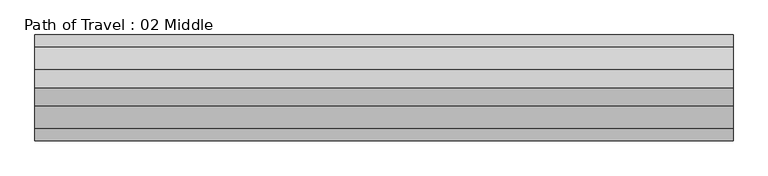
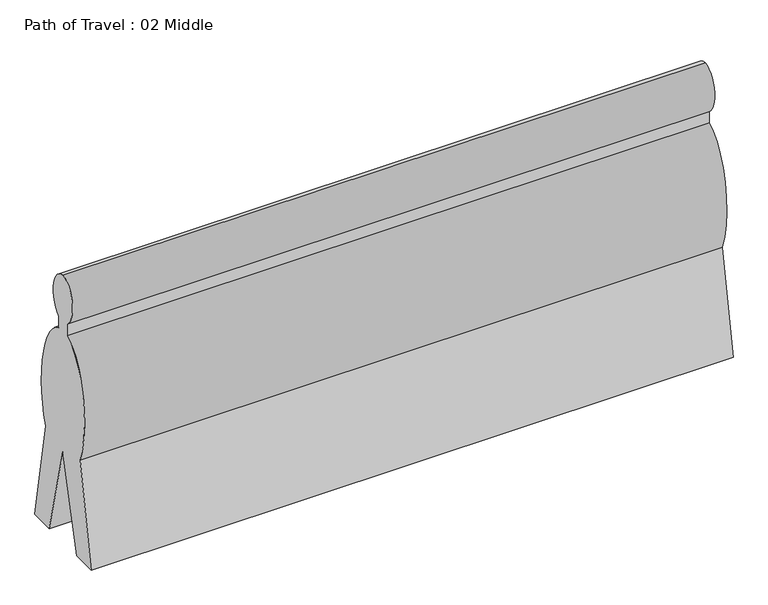
"""IFC4 building model written with IfcOpenShell, lengths in millimetres: proxy geometry, Path of Travel : 02 Middle."""

import ifcopenshell
import ifcopenshell.guid

model = None  # the IFC model being written
_history = None  # IfcOwnerHistory: only IFC2X3 demands one
_inside = {}  # id of a spatial element -> (the spatial element, [elements in it])
_under = {}  # id of a project, library or spatial element -> (it, [spatial elements below it])
_declared = {}  # id of a project -> (the project, [libraries it declares])
_typed = {}  # id of a type object -> (the type object, [elements of that type])
_made_of = {}  # id of a material, layer set ... -> (it, [elements and type objects made of it])


def new_model(schema):
    """Start an empty IFC model of exactly this schema.

    Asked for "IFC4X3", IfcOpenShell would pick the latest addendum, in which some entities
    have other attributes; the version numbers below select the first issue.
    IFC2X3 requires an IfcOwnerHistory on every rooted entity: one is made here for all.
    """
    global model, _history
    if schema == "IFC4X3":
        model = ifcopenshell.file(schema_version=(4, 3, 0, 0))
    else:
        model = ifcopenshell.file(schema=schema)
    _inside.clear()
    _under.clear()
    _declared.clear()
    _typed.clear()
    _made_of.clear()
    _history = None
    if model.schema == "IFC2X3":
        org = make("IfcOrganization", Name="unknown")
        user = make(
            "IfcPersonAndOrganization",
            ThePerson=make("IfcPerson", FamilyName="unknown"),
            TheOrganization=org,
        )
        app = make(
            "IfcApplication",
            ApplicationDeveloper=org,
            Version="unknown",
            ApplicationFullName="unknown",
            ApplicationIdentifier="unknown",
        )
        _history = make(
            "IfcOwnerHistory",
            OwningUser=user,
            OwningApplication=app,
            ChangeAction="ADDED",
            CreationDate=0,
        )
    return model


def make(cls, **values):
    """One entity of the class cls with the attributes given. An attribute that is None is left unset."""
    return model.create_entity(
        cls, **{name: value for name, value in values.items() if value is not None}
    )


def rooted(cls, **values):
    """An entity with a GlobalId (a new one), such as an element, a storey or a relation."""
    return make(cls, GlobalId=ifcopenshell.guid.new(), OwnerHistory=_history, **values)


def si_unit(unit_type, name, prefix=None):
    """IfcSIUnit, for example si_unit("LENGTHUNIT", "METRE", prefix="MILLI")."""
    return make("IfcSIUnit", UnitType=unit_type, Prefix=prefix, Name=name)


def assignment(units):
    """IfcUnitAssignment: the units of a project."""
    return None if units is None else make("IfcUnitAssignment", Units=units)


def point(xyz):
    """IfcCartesianPoint."""
    return None if xyz is None else make("IfcCartesianPoint", Coordinates=xyz)


def direction(xyz):
    """IfcDirection."""
    return None if xyz is None else make("IfcDirection", DirectionRatios=xyz)


def frame(location, z_axis=None, x_axis=None):
    """IfcAxis2Placement3D, a coordinate frame: its origin and axes. An axis left out is left unset."""
    return make(
        "IfcAxis2Placement3D",
        Location=point(location),
        Axis=direction(z_axis),
        RefDirection=direction(x_axis),
    )


def origin():
    """The frame at (0, 0, 0) with its axes left unset."""
    return frame((0.0, 0.0, 0.0))


def place(relative_to, where):
    """IfcLocalPlacement: puts the frame where relative to a parent placement (None: the world)."""
    return make(
        "IfcLocalPlacement", PlacementRelTo=relative_to, RelativePlacement=where
    )


def context(
    kind, dimensions, precision=None, world=None, true_north=None, identifier=None
):
    """IfcGeometricRepresentationContext, for example the 3D "Model" context."""
    return make(
        "IfcGeometricRepresentationContext",
        ContextIdentifier=identifier,
        ContextType=kind,
        CoordinateSpaceDimension=dimensions,
        Precision=precision,
        WorldCoordinateSystem=world,
        TrueNorth=true_north,
    )


def project(units=None, contexts=None):
    """IfcProject with its units and contexts."""
    return rooted(
        "IfcProject",
        Name="project",
        RepresentationContexts=contexts,
        UnitsInContext=assignment(units),
    )


def spatial(cls, under=None, at=None, **own):
    """A site, building, storey or space (cls), placed at a placement, below another one or the project."""
    s = rooted(cls, ObjectPlacement=at, **own)
    if under is not None:
        _under.setdefault(under.id(), (under, []))[1].append(s)
    return s


def ellipse_curve(where, semi_axis1, semi_axis2):
    """IfcEllipse in the frame where."""
    return make(
        "IfcEllipse", Position=where, SemiAxis1=semi_axis1, SemiAxis2=semi_axis2
    )


def trimmed(basis, trim1, trim2, sense, master):
    """IfcTrimmedCurve: the piece of a basis curve between two trims."""
    return make(
        "IfcTrimmedCurve",
        BasisCurve=basis,
        Trim1=trim1,
        Trim2=trim2,
        SenseAgreement=sense,
        MasterRepresentation=master,
    )


def shape(context_of_items, identifier, shape_type, items):
    """IfcShapeRepresentation: the items that make up one representation, for example the "Body"."""
    return make(
        "IfcShapeRepresentation",
        ContextOfItems=context_of_items,
        RepresentationIdentifier=identifier,
        RepresentationType=shape_type,
        Items=items,
    )


def source(mapping_origin, context_of_items, identifier, shape_type, items):
    """IfcRepresentationMap: a shape defined once, which mapped items show again and again."""
    return make(
        "IfcRepresentationMap",
        MappingOrigin=mapping_origin,
        MappedRepresentation=shape(context_of_items, identifier, shape_type, items),
    )


def transform(
    local_origin,
    x_axis=None,
    y_axis=None,
    z_axis=None,
    scale=None,
    scale2=None,
    scale3=None,
    uniform=True,
):
    """IfcCartesianTransformationOperator3D, or its non-uniform kind. x_axis, y_axis, z_axis: its Axis1, 2, 3."""
    if uniform:
        return make(
            "IfcCartesianTransformationOperator3D",
            Axis1=direction(x_axis),
            Axis2=direction(y_axis),
            LocalOrigin=point(local_origin),
            Scale=scale,
            Axis3=direction(z_axis),
        )
    return make(
        "IfcCartesianTransformationOperator3DnonUniform",
        Axis1=direction(x_axis),
        Axis2=direction(y_axis),
        LocalOrigin=point(local_origin),
        Scale=scale,
        Axis3=direction(z_axis),
        Scale2=scale2,
        Scale3=scale3,
    )


def mapped(mapping_source, mapping_target):
    """IfcMappedItem: shows the shape of a source again, moved by a transform."""
    return make(
        "IfcMappedItem", MappingSource=mapping_source, MappingTarget=mapping_target
    )


def made_of(thing, what):
    """Note that an element or type object is made of a material, layer set ...; save() writes the relation."""
    if what is not None:
        _made_of.setdefault(what.id(), (what, []))[1].append(thing)
    return thing


def element(
    cls,
    number,
    at=None,
    inside=None,
    cuts=None,
    type_object=None,
    material=None,
    context=None,
    identifier="Body",
    shape_type=None,
    held_by="IfcProductDefinitionShape",
    body=None,
    shapes=None,
    **own,
):
    """One element of the class cls, such as IfcWall. Its Tag is "e" and its number.

    at: its placement. inside: the storey or other place that contains it. cuts: it is an
    opening in that element (IfcRelVoidsElement). A single representation is given by context,
    identifier, shape_type and body (its items); several are given by shapes. held_by: the class
    of the entity that holds the representations. save() writes the other relations.
    """
    e = rooted(cls, Tag="e%d" % number, ObjectPlacement=at, **own)
    if body is not None:
        shapes = [shape(context, identifier, shape_type, body)]
    if shapes is not None:
        e.Representation = make(held_by, Representations=shapes)
    if inside is not None:
        _inside.setdefault(inside.id(), (inside, []))[1].append(e)
    if cuts is not None:
        rooted(
            "IfcRelVoidsElement", RelatingBuildingElement=cuts, RelatedOpeningElement=e
        )
    if type_object is not None:
        _typed.setdefault(type_object.id(), (type_object, []))[1].append(e)
    return made_of(e, material)


def aggregate(whole, parts):
    """IfcRelAggregates: a whole, such as a stair, and the parts it consists of."""
    return rooted("IfcRelAggregates", RelatingObject=whole, RelatedObjects=parts)


def save(model, path):
    """Write the relations noted so far, then the file.

    IfcRelAggregates (storeys below a building ...), IfcRelContainedInSpatialStructure (elements
    in a storey), IfcRelDefinesByType, IfcRelAssociatesMaterial and IfcRelDeclares: one each for
    every whole, place, type object, material and project.
    """
    for whole, parts in _under.values():
        aggregate(whole, parts)
    for where, things in _inside.values():
        rooted(
            "IfcRelContainedInSpatialStructure",
            RelatedElements=things,
            RelatingStructure=where,
        )
    for kind, things in _typed.values():
        rooted("IfcRelDefinesByType", RelatedObjects=things, RelatingType=kind)
    for what, things in _made_of.values():
        rooted("IfcRelAssociatesMaterial", RelatedObjects=things, RelatingMaterial=what)
    for by, libraries in _declared.values():
        rooted("IfcRelDeclares", RelatingContext=by, RelatedDefinitions=libraries)
    model.write(path)


def plane_surface(at):
    """IfcPlane: the flat surface through the origin of the frame at, square to its z axis."""
    return make("IfcPlane", Position=at)


def extruded_surface(curve, direction_of_extrusion, depth):
    """IfcSurfaceOfLinearExtrusion: the curve pushed along a direction by depth."""
    return make(
        "IfcSurfaceOfLinearExtrusion",
        SweptCurve=make("IfcArbitraryOpenProfileDef", ProfileType="CURVE", Curve=curve),
        ExtrudedDirection=direction(direction_of_extrusion),
        Depth=depth,
    )


def advanced_brep(points, edges, surfaces, faces):
    """IfcAdvancedBrep: a solid bounded by faces that lie on surfaces and meet in shared edges.

    An edge is (start, end): straight between two places in points (the first is 0);
    or (start, end, curve); or (start, end, curve, False) where it runs against its curve.
    A face is (place in surfaces, loops), or (place, loops, False) where it looks against
    its surface's normal. A loop lists edges by number (the first is 1), with a minus sign
    where the edge is run from its end to its start. The first loop is the outer one.
    """
    corners = [point(p) for p in points]
    vertices = [make("IfcVertexPoint", VertexGeometry=c) for c in corners]
    made = []
    for start, end, *more in edges:
        made.append(
            make(
                "IfcEdgeCurve",
                EdgeStart=vertices[start],
                EdgeEnd=vertices[end],
                EdgeGeometry=more[0] if more else make("IfcPolyline", Points=[corners[start], corners[end]]),
                SameSense=more[1] if len(more) > 1 else True,
            )
        )
    hull = []
    for where, loops, *sense in faces:
        bounds = []
        for j, loop in enumerate(loops):
            ring = [make("IfcOrientedEdge", EdgeElement=made[abs(k) - 1], Orientation=k > 0) for k in loop]
            bounds.append(
                make(
                    "IfcFaceOuterBound" if j == 0 else "IfcFaceBound",
                    Bound=make("IfcEdgeLoop", EdgeList=ring),
                    Orientation=True,
                )
            )
        hull.append(make("IfcAdvancedFace", Bounds=bounds, FaceSurface=surfaces[where], SameSense=sense[0] if sense else True))
    return make("IfcAdvancedBrep", Outer=make("IfcClosedShell", CfsFaces=hull))


def path_of_travel_02_middle_3cefd49c(model_context):
    return source(origin(), model_context, "Body", "AdvancedBrep", [
        advanced_brep(
        [(227.5554837, 0.0, 1727.2), (227.5554837, 42.9018657, 1436.6534209), (227.5554837, 42.9018657, 1363.4763406), (227.5554837, 184.1186263, 643.4144547), (227.5554837, 297.5699544, 0.0), (227.5554837, 145.6574193, 0.0), (227.5554837, 0.0, 584.2), (227.5554837, -145.6574193, 0.0), (227.5554837, -297.5699544, 0.0), (227.5554837, -184.1186263, 643.4144547), (227.5554837, -42.9018657, 1363.4763406), (227.5554837, -42.9018657, 1436.6534209), (4159.8758778, 0.0, 1727.2), (4159.8758778, -42.9018657, 1436.6534209), (4159.8758778, -42.9018657, 1363.4763406), (4159.8758778, -184.1186263, 643.4144547), (4159.8758778, -297.5699544, 0.0), (4159.8758778, -145.6574193, 0.0), (4159.8758778, 0.0, 584.2), (4159.8758778, 145.6574193, 0.0), (4159.8758778, 297.5699544, 0.0), (4159.8758778, 184.1186263, 643.4144547), (4159.8758778, 42.9018657, 1363.4763406), (4159.8758778, 42.9018657, 1436.6534209)],
        [
            (0, 1, ellipse_curve(frame((227.5554837, 0.0, 1574.8), z_axis=(-1.0, 0.0, 0.0), x_axis=(0.0, 0.0, 1.0)), 152.4, 101.6)),
            (1, 2),
            (2, 3, ellipse_curve(frame((227.5554837, 0.0, 914.4), z_axis=(-1.0, 0.0, 0.0), x_axis=(0.0, 0.0, -1.0)), 457.2, 228.6)),
            (3, 4),
            (4, 5),
            (5, 6),
            (6, 7),
            (7, 8),
            (8, 9),
            (9, 10, ellipse_curve(frame((227.5554837, 0.0, 914.4), z_axis=(-1.0, 0.0, 0.0), x_axis=(0.0, 0.0, -1.0)), 457.2, 228.6)),
            (10, 11),
            (11, 0, ellipse_curve(frame((227.5554837, 0.0, 1574.8), z_axis=(-1.0, 0.0, 0.0), x_axis=(0.0, 0.0, 1.0)), 152.4, 101.6)),
            (12, 13, ellipse_curve(frame((4159.8758778, 0.0, 1574.8), z_axis=(1.0, 0.0, 0.0), x_axis=(0.0, 0.0, 1.0)), 152.4, 101.6)),
            (13, 14),
            (14, 15, ellipse_curve(frame((4159.8758778, 0.0, 914.4), z_axis=(1.0, 0.0, 0.0), x_axis=(0.0, 0.0, -1.0)), 457.2, 228.6)),
            (15, 16),
            (16, 17),
            (17, 18),
            (18, 19),
            (19, 20),
            (20, 21),
            (21, 22, ellipse_curve(frame((4159.8758778, 0.0, 914.4), z_axis=(1.0, 0.0, 0.0), x_axis=(0.0, 0.0, -1.0)), 457.2, 228.6)),
            (22, 23),
            (23, 12, ellipse_curve(frame((4159.8758778, 0.0, 1574.8), z_axis=(1.0, 0.0, 0.0), x_axis=(0.0, 0.0, 1.0)), 152.4, 101.6)),
            (0, 12),
            (23, 1),
            (22, 2),
            (21, 3),
            (20, 4),
            (19, 5),
            (18, 6),
            (17, 7),
            (16, 8),
            (15, 9),
            (14, 10),
            (13, 11),
        ],
        [
            plane_surface(frame((227.5554837, 0.0, 0.0), z_axis=(-1.0, 0.0, 0.0), x_axis=(0.0, 0.0, 1.0))),
            plane_surface(frame((4159.8758778, 0.0, 0.0), z_axis=(1.0, 0.0, 0.0), x_axis=(0.0, 0.0, 1.0))),
            extruded_surface(trimmed(ellipse_curve(frame((4159.8758778, 0.0, 1574.8), z_axis=(-1.0, 0.0, 0.0), x_axis=(0.0, 0.0, 1.0)), 152.4, 101.6), [point((4159.8758778, 0.0, 1727.2))], [point((4159.8758778, 42.9018657, 1436.6534209))], True, "CARTESIAN"), (-3932.3203941, 0.0, 0.0), 3932.3203941),
            plane_surface(frame((227.5554837, 42.9018657, 1436.6534209), z_axis=(0.0, 1.0, 0.0), x_axis=(1.0, 0.0, 0.0))),
            extruded_surface(trimmed(ellipse_curve(frame((4159.8758778, 0.0, 914.4), z_axis=(-1.0, 0.0, 0.0), x_axis=(0.0, 0.0, -1.0)), 457.2, 228.6), [point((4159.8758778, 42.9018657, 1363.4763406))], [point((4159.8758778, 184.1186263, 643.4144547))], True, "CARTESIAN"), (-3932.3203941, 0.0, 0.0), 3932.3203941),
            plane_surface(frame((227.5554837, 184.1186263, 643.4144547), z_axis=(0.0, 0.9848077530122078, 0.17364817766693205), x_axis=(1.0, 0.0, 0.0))),
            plane_surface(frame((227.5554837, 297.5699544, 0.0), z_axis=(0.0, 0.0, -1.0), x_axis=(1.0, 0.0, 0.0))),
            plane_surface(frame((227.5554837, 145.6574193, 0.0), z_axis=(0.0, -0.9702957262760199, -0.2419218955995739), x_axis=(1.0, 0.0, 0.0))),
            plane_surface(frame((227.5554837, 0.0, 584.2), z_axis=(0.0, 0.9702957262759961, -0.24192189559966923), x_axis=(1.0, 0.0, 0.0))),
            plane_surface(frame((227.5554837, -145.6574193, 0.0), z_axis=(0.0, 0.0, -1.0), x_axis=(1.0, 0.0, 0.0))),
            plane_surface(frame((227.5554837, -297.5699544, 0.0), z_axis=(0.0, -0.984807753012208, 0.17364817766693066), x_axis=(1.0, 0.0, 0.0))),
            extruded_surface(trimmed(ellipse_curve(frame((4159.8758778, 0.0, 914.4), z_axis=(-1.0, 0.0, 0.0), x_axis=(0.0, 0.0, -1.0)), 457.2, 228.6), [point((4159.8758778, -184.1186263, 643.4144547))], [point((4159.8758778, -42.9018657, 1363.4763406))], True, "CARTESIAN"), (-3932.3203941, 0.0, 0.0), 3932.3203941),
            plane_surface(frame((227.5554837, -42.9018657, 1363.4763406), z_axis=(0.0, -1.0, 0.0), x_axis=(1.0, 0.0, 0.0))),
            extruded_surface(trimmed(ellipse_curve(frame((4159.8758778, 0.0, 1574.8), z_axis=(-1.0, 0.0, 0.0), x_axis=(0.0, 0.0, 1.0)), 152.4, 101.6), [point((4159.8758778, -42.9018657, 1436.6534209))], [point((4159.8758778, 0.0, 1727.2))], True, "CARTESIAN"), (-3932.3203941, 0.0, 0.0), 3932.3203941),
        ],
        [
            (0, [[1, 2, 3, 4, 5, 6, 7, 8, 9, 10, 11, 12]]),
            (1, [[13, 14, 15, 16, 17, 18, 19, 20, 21, 22, 23, 24]]),
            (2, [[-1, 25, -24, 26]]),
            (3, [[-2, -26, -23, 27]]),
            (4, [[-3, -27, -22, 28]]),
            (5, [[-4, -28, -21, 29]]),
            (6, [[-5, -29, -20, 30]]),
            (7, [[-6, -30, -19, 31]]),
            (8, [[-7, -31, -18, 32]]),
            (9, [[-8, -32, -17, 33]]),
            (10, [[-9, -33, -16, 34]]),
            (11, [[-10, -34, -15, 35]]),
            (12, [[-11, -35, -14, 36]]),
            (13, [[-12, -36, -13, -25]]),
        ],
    ),
    ])


if __name__ == "__main__":
    model = new_model("IFC4")
    model_context = context("Model", 3, world=origin())
    ifc_project = project(units=[si_unit("LENGTHUNIT", "METRE", prefix="MILLI")], contexts=[model_context])
    site = spatial("IfcSite", under=ifc_project)
    building = spatial("IfcBuilding", under=site)
    placement = place(None, origin())
    path_of_travel_02_middle_shape = path_of_travel_02_middle_3cefd49c(model_context)
    element("IfcBuildingElementProxy", 1, Name="Path of Travel : 02 Middle", ObjectType="Path of Travel : 02 Middle", at=placement, inside=building, context=model_context, shape_type="MappedRepresentation", body=[
        mapped(path_of_travel_02_middle_shape, transform((0.0, 0.0, 0.0), x_axis=(1.0, 0.0, 0.0), y_axis=(0.0, 1.0, 0.0), z_axis=(0.0, 0.0, 1.0))),
    ])
    save(model, "model.ifc")

# Revit data of these elements
# Type "Path of Travel : 02 Middle"
#   Path of Egress [instance default] = 4' - 0"
#   built-in parameter 1001306 [instance default] = 4 (stored number, unit not read)
#   Dot at Start = no
#   Arrow in Middle = yes
#   Arrow at End = no
#   Egress Path = none
# Element 1 (IfcBuildingElementProxy, "Path of Travel : 02 Middle")
#   Path of Egress = 12' - 10.81576"
#   built-in parameter 1001306 = 12.9013 (stored number, unit not read)
#   Materials on its faces: "Egress Path Solid"
# Materials
#   "Egress Path Solid": class "Unassigned", colour RGB 255 128 64, transparency 0.75, Comments = "Rendering appearance not upgraded "
